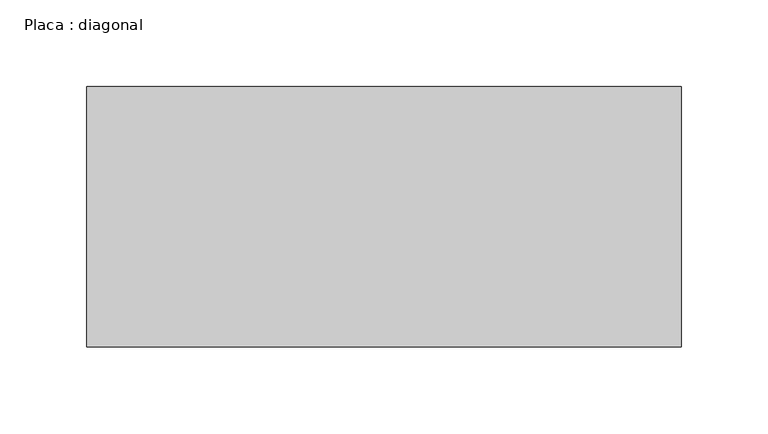
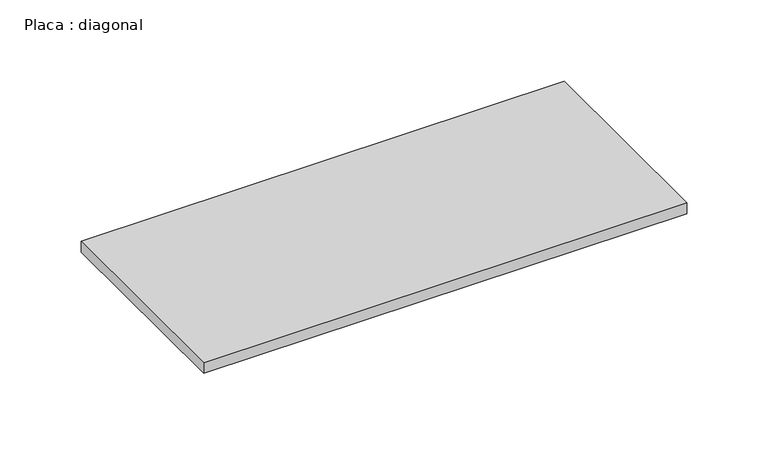
"""IFC4 building model written with IfcOpenShell, lengths in millimetres: beam geometry, Placa : diagonal."""

from ifc_helpers import new_model, si_unit, frame, origin, place, context, project, spatial, polyline, outline, extrude, source, transform, mapped, element, save


def placa_diagonal_d92fe461(model_context):
    return source(origin(), model_context, "Body", "SweptSolid", [
        extrude(outline(polyline([(171.6122376, 75.0), (171.6122376, -75.0), (-170.6977745, -75.0), (-170.6977745, 75.0), (171.6122376, 75.0)])), frame((0.0, 0.0, -4.0), z_axis=(0.0, 0.0, 1.0), x_axis=(1.0, 0.0, 0.0)), (0.0, 0.0, 1.0), 8.0),
    ])


if __name__ == "__main__":
    model = new_model("IFC4")
    model_context = context("Model", 3, world=origin())
    ifc_project = project(units=[si_unit("LENGTHUNIT", "METRE", prefix="MILLI")], contexts=[model_context])
    site = spatial("IfcSite", under=ifc_project)
    building = spatial("IfcBuilding", under=site)
    placement = place(None, origin())
    placa_diagonal_shape = placa_diagonal_d92fe461(model_context)
    element("IfcBeam", 1, ObjectType="Placa : diagonal", at=placement, inside=building, context=model_context, shape_type="MappedRepresentation", body=[
        mapped(placa_diagonal_shape, transform((0.0, 0.0, 0.0), x_axis=(1.0, 0.0, 0.0), y_axis=(0.0, 1.0, 0.0), z_axis=(0.0, 0.0, 1.0))),
    ])
    save(model, "model.ifc")

# Revit data of these elements
# Type "Placa : diagonal"
#   W = 0
#   Length [instance default] = 1.50 m
#   b = 0.15 m
#   d = 0.008 m
#   A = 0 m²
#   Structural Material [instance default] = Aço, 45-345
# Element 1 (IfcBeam, "Placa : diagonal")
#   Materials on its faces: "Aço, 45-345"
# Materials
#   "Aço, 45-345": class "Metal", colour RGB 247 247 247, transparency 0, Description = "Aço 345 MPa", Cost = 0
